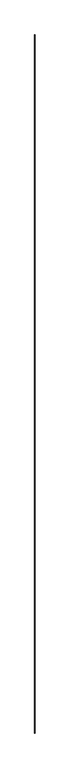
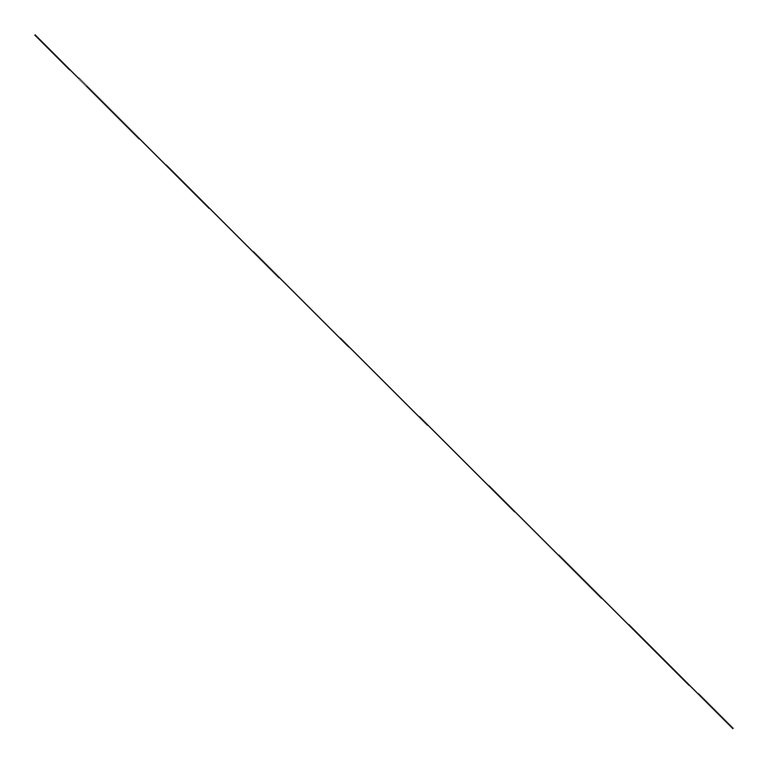
"""IFC4 building model written with IfcOpenShell, lengths in millimetres: proxy geometry, Inner panel:Inner panel:1:Inner panel:1 : Inner panel:Inner panel:300324:2:Inner panel:1:Inner panel:1 : Inner panel:Inner panel:300324:2 : Inner panel:Inner panel:1:Inner panel:1 : Inner panel:Inner panel:300324:300043:4 : Inner panel:Inner panel:1:Inner panel:1 : Inner panel:Inner panel:300324:2:Inner panel:1:Inner panel:1 : Inner panel:Inner panel:300324:2 : Inner panel:Inner panel:1:Inner panel:1 : Inner panel:Inner panel:300324:300043:308120."""

from ifc_helpers import new_model, si_unit, frame, origin, place, context, project, spatial, polyline, outline, extrude, source, transform, mapped, element, save


def generic_models_b7e41361(model_context):
    return source(origin(), model_context, "Body", "SweptSolid", [
        extrude(outline(polyline([(8919.2746389, 566568.2010371), (8901.3141267, 566586.1615493), (8919.2746389, 566604.1220616), (8937.2351512, 566586.1615493), (8919.2746389, 566568.2010371)]), holes=[polyline([(8919.2746389, 566571.5686331), (8933.8675551, 566586.1615493), (8919.2746389, 566600.7544655), (8904.6817227, 566586.1615493), (8919.2746389, 566571.5686331)])]), frame((0.0, -557134.6616705, 0.0), z_axis=(0.0, 1.0, 0.0), x_axis=(0.0, 0.0, 1.0)), (0.0, 0.0, 1.0), 88442.8),
    ])


if __name__ == "__main__":
    model = new_model("IFC4")
    model_context = context("Model", 3, world=origin())
    ifc_project = project(units=[si_unit("LENGTHUNIT", "METRE", prefix="MILLI")], contexts=[model_context])
    site = spatial("IfcSite", under=ifc_project)
    building = spatial("IfcBuilding", under=site)
    placement = place(None, origin())
    generic_models_shape = generic_models_b7e41361(model_context)
    element("IfcBuildingElementProxy", 1, Name="Inner panel:Inner panel:1:Inner panel:1 : Inner panel:Inner panel:300324:2:Inner panel:1:Inner panel:1 : Inner panel:Inner panel:300324:2 : Inner panel:Inner panel:1:Inner panel:1 : Inner panel:Inner panel:300324:300043:4 : Inner panel:Inner panel:1:Inner panel:1 : Inner panel:Inner panel:300324:2:Inner panel:1:Inner panel:1 : Inner panel:Inner panel:300324:2 : Inner panel:Inner panel:1:Inner panel:1 : Inner panel:Inner panel:300324:300043:308120", ObjectType="Inner panel:Inner panel:1:Inner panel:1 : Inner panel:Inner panel:300324:2:Inner panel:1:Inner panel:1 : Inner panel:Inner panel:300324:2 : Inner panel:Inner panel:1:Inner panel:1 : Inner panel:Inner panel:300324:300043:4 : Inner panel:Inner panel:1:Inner panel:1 : Inner panel:Inner panel:300324:2:Inner panel:1:Inner panel:1 : Inner panel:Inner panel:300324:2 : Inner panel:Inner panel:1:Inner panel:1 : Inner panel:Inner panel:300324:300043:308120", at=placement, inside=building, context=model_context, shape_type="MappedRepresentation", body=[
        mapped(generic_models_shape, transform((0.0, 0.0, 0.0), x_axis=(1.0, 0.0, 0.0), y_axis=(0.0, 1.0, 0.0), z_axis=(0.0, 0.0, 1.0))),
    ])
    save(model, "model.ifc")

# Revit data of these elements
# Type "Inner panel:Inner panel:1:Inner panel:1 : Inner panel:Inner panel:300324:2:Inner panel:1:Inner panel:1 : Inner panel:Inner panel:300324:2 : Inner panel:Inner panel:1:Inner panel:1 : Inner panel:Inner panel:300324:300043:4 : Inner panel:Inner panel:1:Inner panel:1 : Inner panel:Inner panel:300324:2:Inner panel:1:Inner panel:1 : Inner panel:Inner panel:300324:2 : Inner panel:Inner panel:1:Inner panel:1 : Inner panel:Inner panel:300324:300043:308120"
#   NameOverride = "Inner panel:Inner panel:1:Inner panel:1 : Inner panel:Inner panel:300324:2:Inner panel:1:Inner panel:1 : Inner panel:Inner panel:300324:2 : Inner panel:Inner panel:1:Inner panel:1 : Inner panel:Inner panel:300324:300043:308120"
#   ObjectTypeOverride = "Inner panel:1:Inner panel:1 : Inner panel:Inner panel:300324:2 : Inner panel:Inner panel:1:Inner panel:1 : Inner panel:Inner panel:300324:300043"
#   Reference = "Inner panel"
#   Tag = "308120"
# Element 1 (IfcBuildingElementProxy, "Inner panel:Inner panel:1:Inner panel:1 : Inner panel:Inner panel:300324:2:Inner panel:1:Inner panel:1 : Inner panel:Inner panel:300324:2 : Inner panel:Inner panel:1:Inner panel:1 : Inner panel:Inner panel:300324:300043:4 : Inner panel:Inner panel:1:Inner panel:1 : Inner panel:Inner panel:300324:2:Inner panel:1:Inner panel:1 : Inner panel:Inner panel:300324:2 : Inner panel:Inner panel:1:Inner panel:1 : Inner panel:Inner panel:300324:300043:308120")
#   Materials on its faces: "SNOW GUARD SYSTEM"
# Materials
#   "SNOW GUARD SYSTEM": class "Generic", colour RGB 223 223 223, transparency 0, Cost = 0
